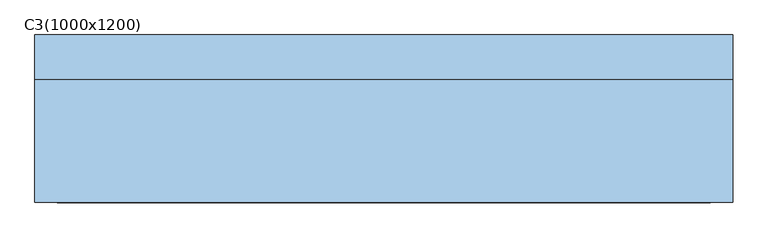
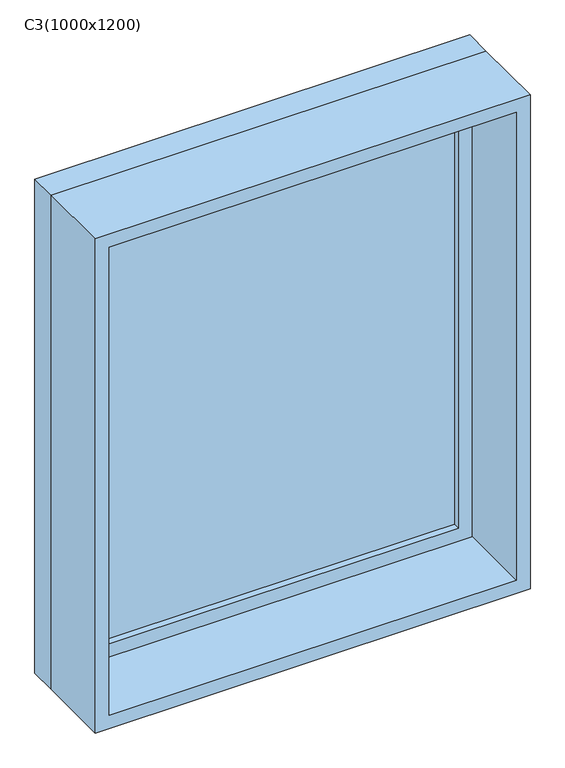
"""IFC4 building model written with IfcOpenShell, lengths in millimetres: window geometry, 固定窗 : C3(1000x1200)."""

import ifcopenshell
import ifcopenshell.guid

model = None  # the IFC model being written
_history = None  # IfcOwnerHistory: only IFC2X3 demands one
_inside = {}  # id of a spatial element -> (the spatial element, [elements in it])
_under = {}  # id of a project, library or spatial element -> (it, [spatial elements below it])
_declared = {}  # id of a project -> (the project, [libraries it declares])
_typed = {}  # id of a type object -> (the type object, [elements of that type])
_made_of = {}  # id of a material, layer set ... -> (it, [elements and type objects made of it])


def new_model(schema):
    """Start an empty IFC model of exactly this schema.

    Asked for "IFC4X3", IfcOpenShell would pick the latest addendum, in which some entities
    have other attributes; the version numbers below select the first issue.
    IFC2X3 requires an IfcOwnerHistory on every rooted entity: one is made here for all.
    """
    global model, _history
    if schema == "IFC4X3":
        model = ifcopenshell.file(schema_version=(4, 3, 0, 0))
    else:
        model = ifcopenshell.file(schema=schema)
    _inside.clear()
    _under.clear()
    _declared.clear()
    _typed.clear()
    _made_of.clear()
    _history = None
    if model.schema == "IFC2X3":
        org = make("IfcOrganization", Name="unknown")
        user = make(
            "IfcPersonAndOrganization",
            ThePerson=make("IfcPerson", FamilyName="unknown"),
            TheOrganization=org,
        )
        app = make(
            "IfcApplication",
            ApplicationDeveloper=org,
            Version="unknown",
            ApplicationFullName="unknown",
            ApplicationIdentifier="unknown",
        )
        _history = make(
            "IfcOwnerHistory",
            OwningUser=user,
            OwningApplication=app,
            ChangeAction="ADDED",
            CreationDate=0,
        )
    return model


def make(cls, **values):
    """One entity of the class cls with the attributes given. An attribute that is None is left unset."""
    return model.create_entity(
        cls, **{name: value for name, value in values.items() if value is not None}
    )


def rooted(cls, **values):
    """An entity with a GlobalId (a new one), such as an element, a storey or a relation."""
    return make(cls, GlobalId=ifcopenshell.guid.new(), OwnerHistory=_history, **values)


def si_unit(unit_type, name, prefix=None):
    """IfcSIUnit, for example si_unit("LENGTHUNIT", "METRE", prefix="MILLI")."""
    return make("IfcSIUnit", UnitType=unit_type, Prefix=prefix, Name=name)


def assignment(units):
    """IfcUnitAssignment: the units of a project."""
    return None if units is None else make("IfcUnitAssignment", Units=units)


def point(xyz):
    """IfcCartesianPoint."""
    return None if xyz is None else make("IfcCartesianPoint", Coordinates=xyz)


def direction(xyz):
    """IfcDirection."""
    return None if xyz is None else make("IfcDirection", DirectionRatios=xyz)


def frame(location, z_axis=None, x_axis=None):
    """IfcAxis2Placement3D, a coordinate frame: its origin and axes. An axis left out is left unset."""
    return make(
        "IfcAxis2Placement3D",
        Location=point(location),
        Axis=direction(z_axis),
        RefDirection=direction(x_axis),
    )


def origin():
    """The frame at (0, 0, 0) with its axes left unset."""
    return frame((0.0, 0.0, 0.0))


def place(relative_to, where):
    """IfcLocalPlacement: puts the frame where relative to a parent placement (None: the world)."""
    return make(
        "IfcLocalPlacement", PlacementRelTo=relative_to, RelativePlacement=where
    )


def context(
    kind, dimensions, precision=None, world=None, true_north=None, identifier=None
):
    """IfcGeometricRepresentationContext, for example the 3D "Model" context."""
    return make(
        "IfcGeometricRepresentationContext",
        ContextIdentifier=identifier,
        ContextType=kind,
        CoordinateSpaceDimension=dimensions,
        Precision=precision,
        WorldCoordinateSystem=world,
        TrueNorth=true_north,
    )


def project(units=None, contexts=None):
    """IfcProject with its units and contexts."""
    return rooted(
        "IfcProject",
        Name="project",
        RepresentationContexts=contexts,
        UnitsInContext=assignment(units),
    )


def spatial(cls, under=None, at=None, **own):
    """A site, building, storey or space (cls), placed at a placement, below another one or the project."""
    s = rooted(cls, ObjectPlacement=at, **own)
    if under is not None:
        _under.setdefault(under.id(), (under, []))[1].append(s)
    return s


def polyline(points):
    """IfcPolyline through the points."""
    return make("IfcPolyline", Points=[point(p) for p in points])


def outline(outer, holes=None, kind="AREA"):
    """IfcArbitraryClosedProfileDef: a profile drawn as a closed curve; with holes, ...WithVoids."""
    if holes is None:
        return make("IfcArbitraryClosedProfileDef", ProfileType=kind, OuterCurve=outer)
    return make(
        "IfcArbitraryProfileDefWithVoids",
        ProfileType=kind,
        OuterCurve=outer,
        InnerCurves=holes,
    )


def extrude(swept, where, along, depth):
    """IfcExtrudedAreaSolid: the profile swept, set in the frame where, extruded along a direction by depth."""
    return make(
        "IfcExtrudedAreaSolid",
        SweptArea=swept,
        Position=where,
        ExtrudedDirection=direction(along),
        Depth=depth,
    )


def shape(context_of_items, identifier, shape_type, items):
    """IfcShapeRepresentation: the items that make up one representation, for example the "Body"."""
    return make(
        "IfcShapeRepresentation",
        ContextOfItems=context_of_items,
        RepresentationIdentifier=identifier,
        RepresentationType=shape_type,
        Items=items,
    )


def source(mapping_origin, context_of_items, identifier, shape_type, items):
    """IfcRepresentationMap: a shape defined once, which mapped items show again and again."""
    return make(
        "IfcRepresentationMap",
        MappingOrigin=mapping_origin,
        MappedRepresentation=shape(context_of_items, identifier, shape_type, items),
    )


def transform(
    local_origin,
    x_axis=None,
    y_axis=None,
    z_axis=None,
    scale=None,
    scale2=None,
    scale3=None,
    uniform=True,
):
    """IfcCartesianTransformationOperator3D, or its non-uniform kind. x_axis, y_axis, z_axis: its Axis1, 2, 3."""
    if uniform:
        return make(
            "IfcCartesianTransformationOperator3D",
            Axis1=direction(x_axis),
            Axis2=direction(y_axis),
            LocalOrigin=point(local_origin),
            Scale=scale,
            Axis3=direction(z_axis),
        )
    return make(
        "IfcCartesianTransformationOperator3DnonUniform",
        Axis1=direction(x_axis),
        Axis2=direction(y_axis),
        LocalOrigin=point(local_origin),
        Scale=scale,
        Axis3=direction(z_axis),
        Scale2=scale2,
        Scale3=scale3,
    )


def mapped(mapping_source, mapping_target):
    """IfcMappedItem: shows the shape of a source again, moved by a transform."""
    return make(
        "IfcMappedItem", MappingSource=mapping_source, MappingTarget=mapping_target
    )


def made_of(thing, what):
    """Note that an element or type object is made of a material, layer set ...; save() writes the relation."""
    if what is not None:
        _made_of.setdefault(what.id(), (what, []))[1].append(thing)
    return thing


def element(
    cls,
    number,
    at=None,
    inside=None,
    cuts=None,
    type_object=None,
    material=None,
    context=None,
    identifier="Body",
    shape_type=None,
    held_by="IfcProductDefinitionShape",
    body=None,
    shapes=None,
    **own,
):
    """One element of the class cls, such as IfcWall. Its Tag is "e" and its number.

    at: its placement. inside: the storey or other place that contains it. cuts: it is an
    opening in that element (IfcRelVoidsElement). A single representation is given by context,
    identifier, shape_type and body (its items); several are given by shapes. held_by: the class
    of the entity that holds the representations. save() writes the other relations.
    """
    e = rooted(cls, Tag="e%d" % number, ObjectPlacement=at, **own)
    if body is not None:
        shapes = [shape(context, identifier, shape_type, body)]
    if shapes is not None:
        e.Representation = make(held_by, Representations=shapes)
    if inside is not None:
        _inside.setdefault(inside.id(), (inside, []))[1].append(e)
    if cuts is not None:
        rooted(
            "IfcRelVoidsElement", RelatingBuildingElement=cuts, RelatedOpeningElement=e
        )
    if type_object is not None:
        _typed.setdefault(type_object.id(), (type_object, []))[1].append(e)
    return made_of(e, material)


def aggregate(whole, parts):
    """IfcRelAggregates: a whole, such as a stair, and the parts it consists of."""
    return rooted("IfcRelAggregates", RelatingObject=whole, RelatedObjects=parts)


def save(model, path):
    """Write the relations noted so far, then the file.

    IfcRelAggregates (storeys below a building ...), IfcRelContainedInSpatialStructure (elements
    in a storey), IfcRelDefinesByType, IfcRelAssociatesMaterial and IfcRelDeclares: one each for
    every whole, place, type object, material and project.
    """
    for whole, parts in _under.values():
        aggregate(whole, parts)
    for where, things in _inside.values():
        rooted(
            "IfcRelContainedInSpatialStructure",
            RelatedElements=things,
            RelatingStructure=where,
        )
    for kind, things in _typed.values():
        rooted("IfcRelDefinesByType", RelatedObjects=things, RelatingType=kind)
    for what, things in _made_of.values():
        rooted("IfcRelAssociatesMaterial", RelatedObjects=things, RelatingMaterial=what)
    for by, libraries in _declared.values():
        rooted("IfcRelDeclares", RelatingContext=by, RelatedDefinitions=libraries)
    model.write(path)


def c3_1000x1200_4273239b(model_context):
    return source(origin(), model_context, "Body", "SweptSolid", [
        extrude(outline(polyline([(398.4, 71.425), (-474.6, 71.425), (-474.6, 84.125), (398.4, 84.125), (398.4, 71.425)])), frame((0.0, 0.0, 963.5), z_axis=(0.0, 0.0, 1.0), x_axis=(1.0, 0.0, 0.0)), (0.0, 0.0, 1.0), 1073.0),
        extrude(outline(polyline([(2080.95, -519.05), (919.05, -519.05), (919.05, 442.85), (2080.95, 442.85), (2080.95, -519.05)]), holes=[polyline([(2036.5, -474.6), (2036.5, 398.4), (963.5, 398.4), (963.5, -474.6), (2036.5, -474.6)])]), frame((0.0, 55.55, 0.0), z_axis=(0.0, 1.0, 0.0), x_axis=(0.0, 0.0, 1.0)), (0.0, 0.0, 1.0), 44.45),
        extrude(outline(polyline([(2100.0, -538.1), (900.0, -538.1), (900.0, 461.9), (2100.0, 461.9), (2100.0, -538.1)]), holes=[polyline([(2068.25, -506.35), (2068.25, 430.15), (931.75, 430.15), (931.75, -506.35), (2068.25, -506.35)])]), frame((0.0, -120.0, 0.0), z_axis=(0.0, 1.0, 0.0), x_axis=(0.0, 0.0, 1.0)), (0.0, 0.0, 1.0), 175.55),
        extrude(outline(polyline([(2100.0, 461.9), (2100.0, -538.1), (900.0, -538.1), (900.0, 461.9), (2100.0, 461.9)]), holes=[polyline([(2080.95, 442.85), (919.05, 442.85), (919.05, -519.05), (2080.95, -519.05), (2080.95, 442.85)])]), frame((0.0, 55.55, 0.0), z_axis=(0.0, 1.0, 0.0), x_axis=(0.0, 0.0, 1.0)), (0.0, 0.0, 1.0), 64.45),
    ])


if __name__ == "__main__":
    model = new_model("IFC4")
    model_context = context("Model", 3, world=origin())
    ifc_project = project(units=[si_unit("LENGTHUNIT", "METRE", prefix="MILLI")], contexts=[model_context])
    site = spatial("IfcSite", under=ifc_project)
    building = spatial("IfcBuilding", under=site)
    placement = place(None, origin())
    c3_1000x1200_shape = c3_1000x1200_4273239b(model_context)
    element("IfcWindow", 1, ObjectType="固定窗 : C3(1000x1200)", at=placement, inside=building, context=model_context, shape_type="MappedRepresentation", body=[
        mapped(c3_1000x1200_shape, transform((0.0, 0.0, 0.0), x_axis=(1.0, 0.0, 0.0), y_axis=(0.0, 1.0, 0.0), z_axis=(0.0, 0.0, 1.0))),
    ])
    save(model, "model.ifc")

# Revit data of these elements
# Type "固定窗 : C3(1000x1200)"
#   Type Mark = "C1516"
#   Construction Type Id = "SGL"
#   Analytic Construction = "大型单层玻璃窗"
#   Visual Light Transmittance = 0.9
#   Solar Heat Gain Coefficient = 0.86
#   Rough Width = 1000 mm
#   Rough Height = 1200 mm
#   Heat Transfer Coefficient (U) = 5.5617 W/(m²·K)
#   Height = 1200 mm
#   默认窗台高度 = 900 mm
#   Width = 1000 mm
#   窗嵌入 = 20 mm
#   高窗平面 [instance default] = no
#   通用窗平面 [instance default] = yes
#   玻璃 = none
#   框架材质 = none
#   Wall Closure = (empty or 0)
# Element 1 (IfcWindow, "固定窗 : C3(1000x1200)")
#   Materials on its faces: "玻璃"
# Materials
#   "玻璃": class "玻璃", colour RGB 0 128 192, transparency 0.9, Description = "钠钙玻璃", Cost = 0
